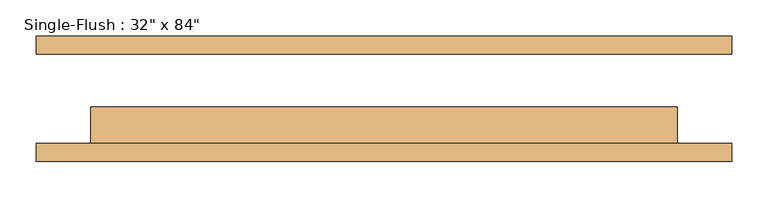
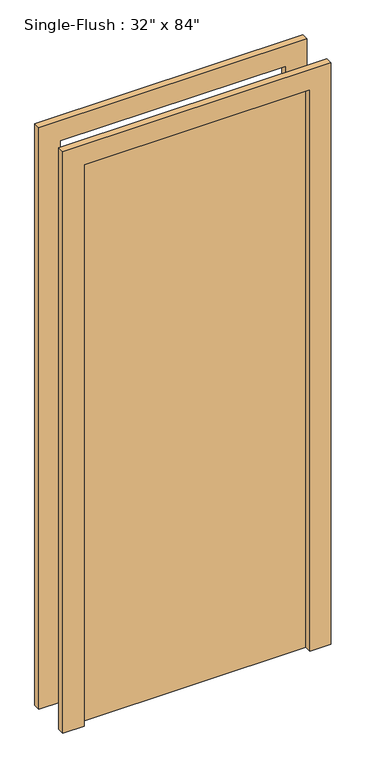
"""IFC4 building model written with IfcOpenShell, lengths in millimetres: door geometry."""

from ifc_helpers import new_model, si_unit, frame, origin, origin_with_axes, place, context, project, spatial, polyline, outline, extrude, source, transform, mapped, element, save


def door_d21431a2(model_context):
    return source(origin(), model_context, "Body", "SweptSolid", [
        extrude(outline(polyline([(2209.8, -482.6), (0.0, -482.6), (0.0, -406.4), (2133.6, -406.4), (2133.6, 406.4), (0.0, 406.4), (0.0, 482.6), (2209.8, 482.6), (2209.8, -482.6)])), frame((0.0, -87.3125, 0.0), z_axis=(0.0, 1.0, 0.0), x_axis=(0.0, 0.0, 1.0)), (0.0, 0.0, 1.0), 25.4),
        extrude(outline(polyline([(2209.8, 482.6), (2209.8, -482.6), (0.0, -482.6), (0.0, -406.4), (2133.6, -406.4), (2133.6, 406.4), (0.0, 406.4), (0.0, 482.6), (2209.8, 482.6)])), frame((0.0, 61.9125, 0.0), z_axis=(0.0, 1.0, 0.0), x_axis=(0.0, 0.0, 1.0)), (0.0, 0.0, 1.0), 25.4),
        extrude(outline(polyline([(406.4, -11.1125), (406.4, -61.9125), (-406.4, -61.9125), (-406.4, -11.1125), (406.4, -11.1125)])), origin_with_axes(), (0.0, 0.0, 1.0), 2133.6),
    ])


if __name__ == "__main__":
    model = new_model("IFC4")
    model_context = context("Model", 3, world=origin())
    ifc_project = project(units=[si_unit("LENGTHUNIT", "METRE", prefix="MILLI")], contexts=[model_context])
    site = spatial("IfcSite", under=ifc_project)
    building = spatial("IfcBuilding", under=site)
    placement = place(None, origin())
    door_shape = door_d21431a2(model_context)
    element("IfcDoor", 1, ObjectType="Single-Flush : 32\" x 84\"", at=placement, inside=building, context=model_context, shape_type="MappedRepresentation", body=[
        mapped(door_shape, transform((0.0, 0.0, 0.0), x_axis=(1.0, 0.0, 0.0), y_axis=(0.0, 1.0, 0.0), z_axis=(0.0, 0.0, 1.0))),
    ])
    save(model, "model.ifc")

# Revit data of these elements
# Type "Single-Flush : 32\" x 84\""
#   Type Mark = "3"
#   Assembly Code = "C1020"
#   Thickness = 0' - 2"
#   Height = 7' - 0"
#   Trim Projection Ext = 0' - 1"
#   Trim Projection Int = 0' - 1"
#   Trim Width = 0' - 3"
#   Width = 2' - 8"
#   Door Material = Door - Panel
#   Frame Material = Door - Frame
#   Function = (empty or 0)
#   Wall Closure = (empty or 0)
# Element 1 (IfcDoor, "Single-Flush : 32\" x 84\"")
#   Materials on its faces: "Door - Frame", "Door - Panel"
# Materials
#   "Door - Panel": class "Wood", colour RGB 114 82 51, transparency 0
#   "Door - Frame": class "Miscellaneous", colour RGB 153 76 43, transparency 0
